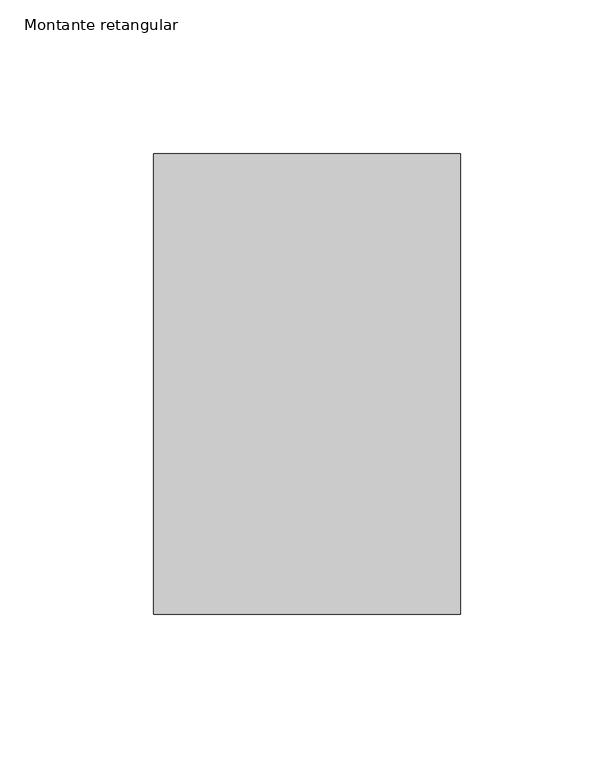
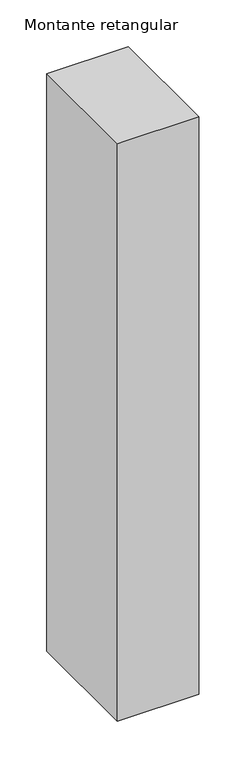
"""IFC4 building model written with IfcOpenShell, lengths in millimetres: member geometry, Montante retangular : CC_100 X 150  mm."""

from ifc_helpers import new_model, si_unit, frame, origin, place, context, project, spatial, polyline, outline, extrude, source, transform, mapped, element, save


def montante_retangular_ab766952(model_context):
    return source(origin(), model_context, "Body", "SweptSolid", [
        extrude(outline(polyline([(50.0, 75.0), (50.0, -75.0), (-50.0, -75.0), (-50.0, 75.0), (50.0, 75.0)])), frame((0.0, 0.0, -750.0), z_axis=(0.0, 0.0, 1.0), x_axis=(1.0, 0.0, 0.0)), (0.0, 0.0, 1.0), 750.0),
    ])


if __name__ == "__main__":
    model = new_model("IFC4")
    model_context = context("Model", 3, world=origin())
    ifc_project = project(units=[si_unit("LENGTHUNIT", "METRE", prefix="MILLI")], contexts=[model_context])
    site = spatial("IfcSite", under=ifc_project)
    building = spatial("IfcBuilding", under=site)
    placement = place(None, origin())
    montante_retangular_shape = montante_retangular_ab766952(model_context)
    element("IfcMember", 1, ObjectType="Montante retangular : CC_100 X 150  mm", at=placement, inside=building, context=model_context, shape_type="MappedRepresentation", body=[
        mapped(montante_retangular_shape, transform((0.0, 0.0, 0.0), x_axis=(1.0, 0.0, 0.0), y_axis=(0.0, 1.0, 0.0), z_axis=(0.0, 0.0, 1.0))),
    ])
    save(model, "model.ifc")

# Revit data of these elements
# Type "Montante retangular : CC_100 X 150  mm"
#   built-in parameter 1007304 = 0.492126 (stored number, unit not read)
#   built-in parameter 1007301 = 0.164042 (stored number, unit not read)
#   built-in parameter 1007300 = 0.164042 (stored number, unit not read)
# Element 1 (IfcMember, "Montante retangular : CC_100 X 150  mm")
#   Materials on its faces: ".ALUMÍNIO"
# Materials
#   ".ALUMÍNIO": class "CC_METAIS", colour RGB 244 244 244, transparency 0, Description = "Material alumínio", Cost = 0
